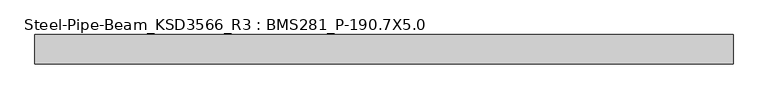
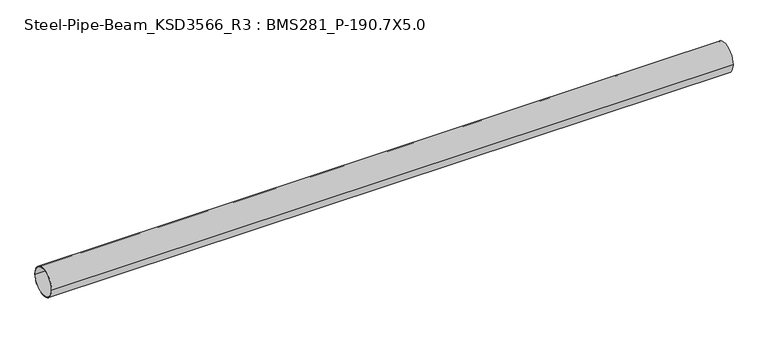
"""IFC4 building model written with IfcOpenShell, lengths in millimetres: member geometry, Steel-Pipe-Beam_KSD3566_R3 : BMS281_P-190.7X5.0."""

from ifc_helpers import new_model, si_unit, point, frame, origin, origin_2d, place, context, project, spatial, circle_curve, trimmed, segment, composite_curve, outline, extrude, source, transform, mapped, element, save


def steel_pipe_beam_ksd3566_r3_bms281_p_190_7x5_0_a82de067(model_context):
    return source(origin(), model_context, "Body", "SweptSolid", [
        extrude(outline(composite_curve([segment(trimmed(circle_curve(origin_2d(), 95.35), [point((-95.35, 0.0))], [point((95.35, 0.0))], False, "CARTESIAN"), True, "CONTINUOUS"), segment(trimmed(circle_curve(origin_2d(), 95.35), [point((95.35, 0.0))], [point((-95.35, 0.0))], False, "CARTESIAN"), True, "CONTINUOUS")], self_intersect=False), holes=[composite_curve([segment(trimmed(circle_curve(origin_2d(), 90.35), [point((90.35, 0.0))], [point((-90.35, 0.0))], True, "CARTESIAN"), True, "CONTINUOUS"), segment(trimmed(circle_curve(origin_2d(), 90.35), [point((-90.35, 0.0))], [point((90.35, 0.0))], True, "CARTESIAN"), True, "CONTINUOUS")], self_intersect=False)]), frame((-2305.4023922, 0.0, 0.0), z_axis=(1.0, 0.0, 0.0), x_axis=(0.0, 1.0, 0.0)), (0.0, 0.0, 1.0), 4533.0400738),
    ])


if __name__ == "__main__":
    model = new_model("IFC4")
    model_context = context("Model", 3, world=origin())
    ifc_project = project(units=[si_unit("LENGTHUNIT", "METRE", prefix="MILLI")], contexts=[model_context])
    site = spatial("IfcSite", under=ifc_project)
    building = spatial("IfcBuilding", under=site)
    placement = place(None, origin())
    steel_pipe_beam_ksd3566_r3_bms281_p_190_7x5_0_shape = steel_pipe_beam_ksd3566_r3_bms281_p_190_7x5_0_a82de067(model_context)
    element("IfcMember", 1, ObjectType="Steel-Pipe-Beam_KSD3566_R3 : BMS281_P-190.7X5.0", at=placement, inside=building, context=model_context, shape_type="MappedRepresentation", body=[
        mapped(steel_pipe_beam_ksd3566_r3_bms281_p_190_7x5_0_shape, transform((0.0, 0.0, 0.0), x_axis=(1.0, 0.0, 0.0), y_axis=(0.0, 1.0, 0.0), z_axis=(0.0, 0.0, 1.0))),
    ])
    save(model, "model.ifc")

# Revit data of these elements
# Type "Steel-Pipe-Beam_KSD3566_R3 : BMS281_P-190.7X5.0"
#   Keynote = "P-190.7X5.0"
#   SteelWeight = "Light"
#   t = 0.0050 m
#   Surface Area = 0.599102 m²/m
#   Section Area = 29.1697 cm²
#   Mass per Unit Length = 22.8982 kg/m
#   Length [instance default] = 1.5000 m
#   D = 0.1907 m
#   hec_material4 [instance default] = none
#   hec_material3 [instance default] = none
#   hec_material2 [instance default] = none
#   hec_material1 [instance default] = none
#   Structural Material [instance default] = Steel, 45-345
#   Assembly Code = ""
# Element 1 (IfcMember, "Steel-Pipe-Beam_KSD3566_R3 : BMS281_P-190.7X5.0")
#   Structural Material = none
# Materials
#   "Steel, 45-345": class "Metal", colour RGB 189 187 185, transparency 0, Description = "Steel 345 MPa", Cost = 0
